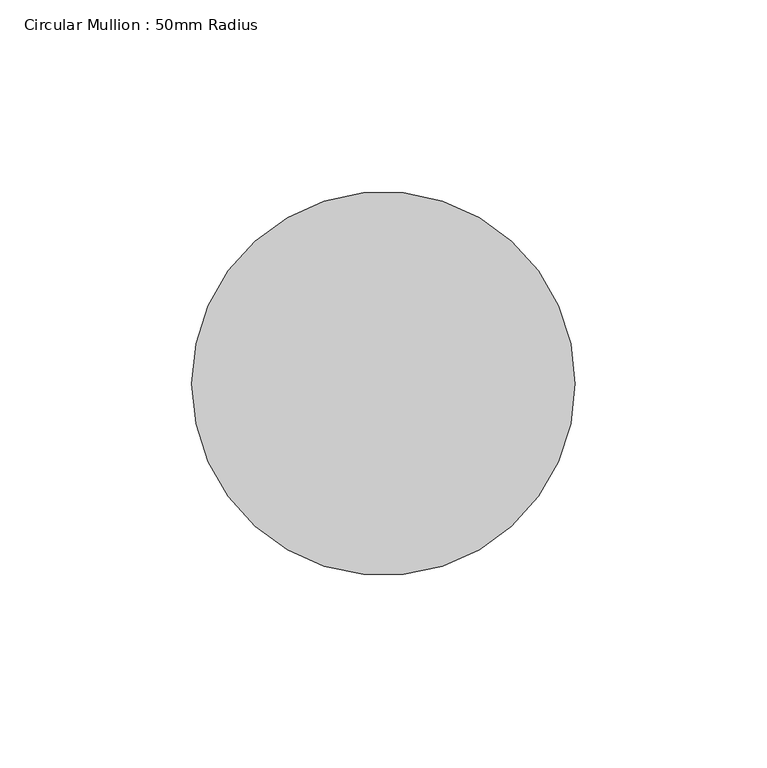
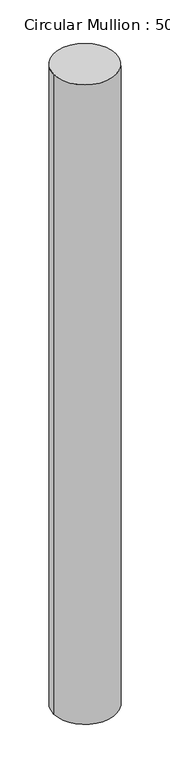
"""IFC4 building model written with IfcOpenShell, lengths in millimetres: member geometry, Circular Mullion : 50mm Radius."""

from ifc_helpers import new_model, si_unit, point, frame, origin, origin_2d, place, context, project, spatial, circle_curve, trimmed, segment, composite_curve, outline, extrude, source, transform, mapped, element, save


def circular_mullion_50mm_radius_b281c513(model_context):
    return source(origin(), model_context, "Body", "SweptSolid", [
        extrude(outline(composite_curve([segment(trimmed(circle_curve(origin_2d(), 50.0), [point((50.0, 0.0))], [point((-50.0, 0.0))], False, "CARTESIAN"), True, "CONTINUOUS"), segment(trimmed(circle_curve(origin_2d(), 50.0), [point((-50.0, 0.0))], [point((50.0, 0.0))], False, "CARTESIAN"), True, "CONTINUOUS")], self_intersect=False)), frame((0.0, 0.0, -1085.131475), z_axis=(0.0, 0.0, 1.0), x_axis=(1.0, 0.0, 0.0)), (0.0, 0.0, 1.0), 1085.131475),
    ])


if __name__ == "__main__":
    model = new_model("IFC4")
    model_context = context("Model", 3, world=origin())
    ifc_project = project(units=[si_unit("LENGTHUNIT", "METRE", prefix="MILLI")], contexts=[model_context])
    site = spatial("IfcSite", under=ifc_project)
    building = spatial("IfcBuilding", under=site)
    placement = place(None, origin())
    circular_mullion_50mm_radius_shape = circular_mullion_50mm_radius_b281c513(model_context)
    element("IfcMember", 1, ObjectType="Circular Mullion : 50mm Radius", at=placement, inside=building, context=model_context, shape_type="MappedRepresentation", body=[
        mapped(circular_mullion_50mm_radius_shape, transform((0.0, 0.0, 0.0), x_axis=(1.0, 0.0, 0.0), y_axis=(0.0, 1.0, 0.0), z_axis=(0.0, 0.0, 1.0))),
    ])
    save(model, "model.ifc")

# Revit data of these elements
# Type "Circular Mullion : 50mm Radius"
#   built-in parameter 1007350 = 0.164042 (stored number, unit not read)
# Element 1 (IfcMember, "Circular Mullion : 50mm Radius")
#   Materials on its faces: "Aluminium"
# Materials
#   "Aluminium": class "Metal", colour RGB 247 247 247, transparency 0, Description = "Aluminium 6061", Cost = 0
